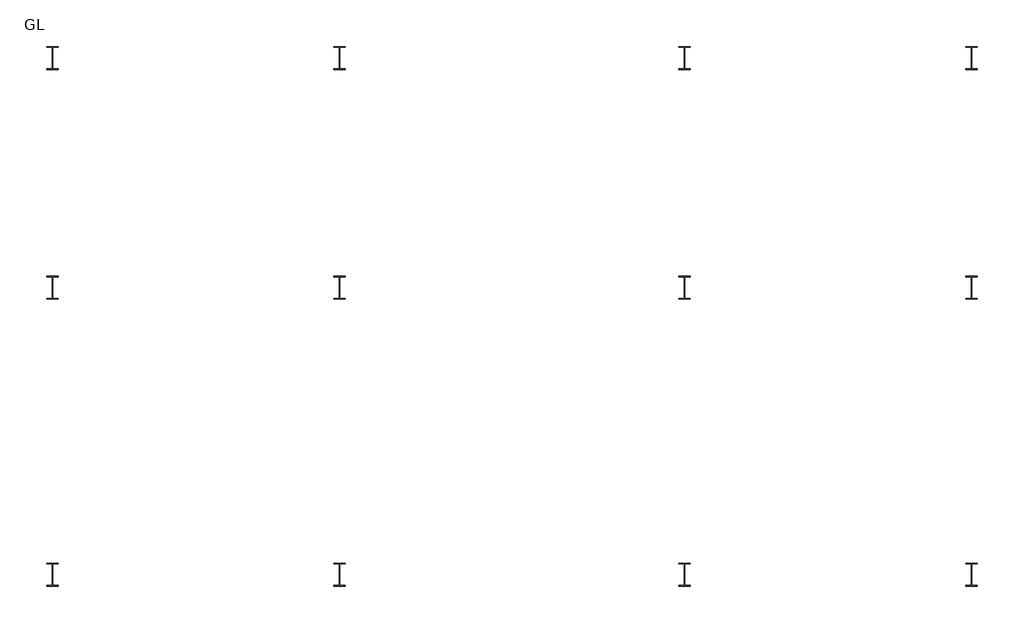
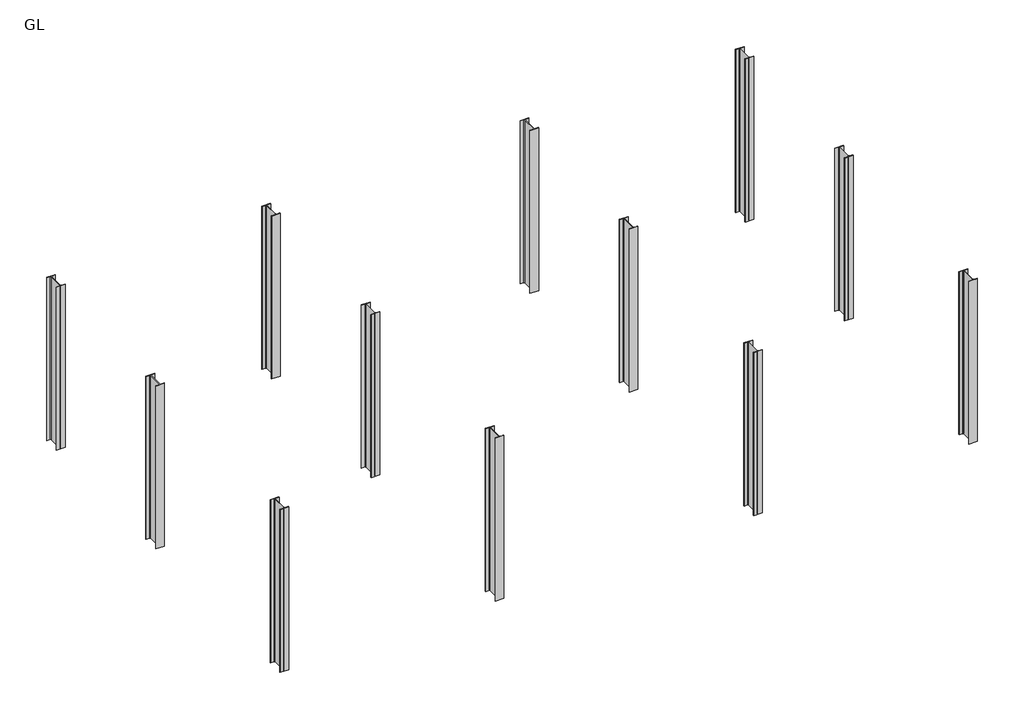
# One storey: 12 columns.
"""IFC4 building model written with IfcOpenShell, lengths in millimetres."""

from ifc_helpers import new_model, si_unit, point, frame_2d, origin, origin_with_axes, place, context, project, spatial, polyline, circle_curve, trimmed, segment, composite_curve, outline, extrude, element, save

model = new_model("IFC4")

# Units and contexts
model_context = context("Model", 3, world=origin())
ifc_project = project(units=[si_unit("LENGTHUNIT", "METRE", prefix="MILLI")], contexts=[model_context])

# Site, building, storey
site = spatial("IfcSite", under=ifc_project)
building = spatial("IfcBuilding", under=site)
storey = spatial("IfcBuildingStorey", under=building, Name="GL", Elevation=-0.0381366)

# Columns
placement = place(None, origin())
element("IfcColumn", 1, ObjectType="Steel Column_H_KSD3502 : H_SC_AR_S01_H-400x200x8x13", at=placement, inside=storey, context=model_context, shape_type="SweptSolid", body=[
    extrude(outline(composite_curve([segment(polyline([(100.0, 200.0), (100.0, 187.0), (20.0, 187.0)]), True, "CONTINUOUS"), segment(trimmed(circle_curve(frame_2d((20.0, 171.0)), 16.0), [point((20.0, 187.0))], [point((4.0, 171.0))], True, "CARTESIAN"), True, "CONTINUOUS"), segment(polyline([(4.0, 171.0), (4.0, -171.0)]), True, "CONTINUOUS"), segment(trimmed(circle_curve(frame_2d((20.0, -171.0)), 16.0), [point((4.0, -171.0))], [point((20.0, -187.0))], True, "CARTESIAN"), True, "CONTINUOUS"), segment(polyline([(20.0, -187.0), (100.0, -187.0), (100.0, -200.0), (-100.0, -200.0), (-100.0, -187.0), (-20.0, -187.0)]), True, "CONTINUOUS"), segment(trimmed(circle_curve(frame_2d((-20.0, -171.0)), 16.0), [point((-20.0, -187.0))], [point((-4.0, -171.0))], True, "CARTESIAN"), True, "CONTINUOUS"), segment(polyline([(-4.0, -171.0), (-4.0, 171.0)]), True, "CONTINUOUS"), segment(trimmed(circle_curve(frame_2d((-20.0, 171.0)), 16.0), [point((-4.0, 171.0))], [point((-20.0, 187.0))], True, "CARTESIAN"), True, "CONTINUOUS"), segment(polyline([(-20.0, 187.0), (-100.0, 187.0), (-100.0, 200.0), (100.0, 200.0)]), True, "CONTINUOUS")], self_intersect=False)), origin_with_axes(), (0.0, 0.0, 1.0), 4000.0),
])
element("IfcColumn", 2, ObjectType="Steel Column_H_KSD3502 : H_SC_AR_S01_H-400x200x8x13", at=placement, inside=storey, context=model_context, shape_type="SweptSolid", body=[
    extrude(outline(composite_curve([segment(polyline([(5100.0, 200.0), (5100.0, 187.0), (5020.0, 187.0)]), True, "CONTINUOUS"), segment(trimmed(circle_curve(frame_2d((5020.0, 171.0)), 16.0), [point((5020.0, 187.0))], [point((5004.0, 171.0))], True, "CARTESIAN"), True, "CONTINUOUS"), segment(polyline([(5004.0, 171.0), (5004.0, -171.0)]), True, "CONTINUOUS"), segment(trimmed(circle_curve(frame_2d((5020.0, -171.0)), 16.0), [point((5004.0, -171.0))], [point((5020.0, -187.0))], True, "CARTESIAN"), True, "CONTINUOUS"), segment(polyline([(5020.0, -187.0), (5100.0, -187.0), (5100.0, -200.0), (4900.0, -200.0), (4900.0, -187.0), (4980.0, -187.0)]), True, "CONTINUOUS"), segment(trimmed(circle_curve(frame_2d((4980.0, -171.0)), 16.0), [point((4980.0, -187.0))], [point((4996.0, -171.0))], True, "CARTESIAN"), True, "CONTINUOUS"), segment(polyline([(4996.0, -171.0), (4996.0, 171.0)]), True, "CONTINUOUS"), segment(trimmed(circle_curve(frame_2d((4980.0, 171.0)), 16.0), [point((4996.0, 171.0))], [point((4980.0, 187.0))], True, "CARTESIAN"), True, "CONTINUOUS"), segment(polyline([(4980.0, 187.0), (4900.0, 187.0), (4900.0, 200.0), (5100.0, 200.0)]), True, "CONTINUOUS")], self_intersect=False)), origin_with_axes(), (0.0, 0.0, 1.0), 4000.0),
])
element("IfcColumn", 3, ObjectType="Steel Column_H_KSD3502 : H_SC_AR_S01_H-400x200x8x13", at=placement, inside=storey, context=model_context, shape_type="SweptSolid", body=[
    extrude(outline(composite_curve([segment(polyline([(11100.0, 200.0), (11100.0, 187.0), (11020.0, 187.0)]), True, "CONTINUOUS"), segment(trimmed(circle_curve(frame_2d((11020.0, 171.0)), 16.0), [point((11020.0, 187.0))], [point((11004.0, 171.0))], True, "CARTESIAN"), True, "CONTINUOUS"), segment(polyline([(11004.0, 171.0), (11004.0, -171.0)]), True, "CONTINUOUS"), segment(trimmed(circle_curve(frame_2d((11020.0, -171.0)), 16.0), [point((11004.0, -171.0))], [point((11020.0, -187.0))], True, "CARTESIAN"), True, "CONTINUOUS"), segment(polyline([(11020.0, -187.0), (11100.0, -187.0), (11100.0, -200.0), (10900.0, -200.0), (10900.0, -187.0), (10980.0, -187.0)]), True, "CONTINUOUS"), segment(trimmed(circle_curve(frame_2d((10980.0, -171.0)), 16.0), [point((10980.0, -187.0))], [point((10996.0, -171.0))], True, "CARTESIAN"), True, "CONTINUOUS"), segment(polyline([(10996.0, -171.0), (10996.0, 171.0)]), True, "CONTINUOUS"), segment(trimmed(circle_curve(frame_2d((10980.0, 171.0)), 16.0), [point((10996.0, 171.0))], [point((10980.0, 187.0))], True, "CARTESIAN"), True, "CONTINUOUS"), segment(polyline([(10980.0, 187.0), (10900.0, 187.0), (10900.0, 200.0), (11100.0, 200.0)]), True, "CONTINUOUS")], self_intersect=False)), origin_with_axes(), (0.0, 0.0, 1.0), 4000.0),
])
element("IfcColumn", 4, ObjectType="Steel Column_H_KSD3502 : H_SC_AR_S01_H-400x200x8x13", at=placement, inside=storey, context=model_context, shape_type="SweptSolid", body=[
    extrude(outline(composite_curve([segment(polyline([(16100.0, 200.0), (16100.0, 187.0), (16020.0, 187.0)]), True, "CONTINUOUS"), segment(trimmed(circle_curve(frame_2d((16020.0, 171.0)), 16.0), [point((16020.0, 187.0))], [point((16004.0, 171.0))], True, "CARTESIAN"), True, "CONTINUOUS"), segment(polyline([(16004.0, 171.0), (16004.0, -171.0)]), True, "CONTINUOUS"), segment(trimmed(circle_curve(frame_2d((16020.0, -171.0)), 16.0), [point((16004.0, -171.0))], [point((16020.0, -187.0))], True, "CARTESIAN"), True, "CONTINUOUS"), segment(polyline([(16020.0, -187.0), (16100.0, -187.0), (16100.0, -200.0), (15900.0, -200.0), (15900.0, -187.0), (15980.0, -187.0)]), True, "CONTINUOUS"), segment(trimmed(circle_curve(frame_2d((15980.0, -171.0)), 16.0), [point((15980.0, -187.0))], [point((15996.0, -171.0))], True, "CARTESIAN"), True, "CONTINUOUS"), segment(polyline([(15996.0, -171.0), (15996.0, 171.0)]), True, "CONTINUOUS"), segment(trimmed(circle_curve(frame_2d((15980.0, 171.0)), 16.0), [point((15996.0, 171.0))], [point((15980.0, 187.0))], True, "CARTESIAN"), True, "CONTINUOUS"), segment(polyline([(15980.0, 187.0), (15900.0, 187.0), (15900.0, 200.0), (16100.0, 200.0)]), True, "CONTINUOUS")], self_intersect=False)), origin_with_axes(), (0.0, 0.0, 1.0), 4000.0),
])
element("IfcColumn", 5, ObjectType="Steel Column_H_KSD3502 : H_SC_AR_S01_H-400x200x8x13", at=placement, inside=storey, context=model_context, shape_type="SweptSolid", body=[
    extrude(outline(composite_curve([segment(polyline([(100.0, 5200.0), (100.0, 5187.0), (20.0, 5187.0)]), True, "CONTINUOUS"), segment(trimmed(circle_curve(frame_2d((20.0, 5171.0)), 16.0), [point((20.0, 5187.0))], [point((4.0, 5171.0))], True, "CARTESIAN"), True, "CONTINUOUS"), segment(polyline([(4.0, 5171.0), (4.0, 4829.0)]), True, "CONTINUOUS"), segment(trimmed(circle_curve(frame_2d((20.0, 4829.0)), 16.0), [point((4.0, 4829.0))], [point((20.0, 4813.0))], True, "CARTESIAN"), True, "CONTINUOUS"), segment(polyline([(20.0, 4813.0), (100.0, 4813.0), (100.0, 4800.0), (-100.0, 4800.0), (-100.0, 4813.0), (-20.0, 4813.0)]), True, "CONTINUOUS"), segment(trimmed(circle_curve(frame_2d((-20.0, 4829.0)), 16.0), [point((-20.0, 4813.0))], [point((-4.0, 4829.0))], True, "CARTESIAN"), True, "CONTINUOUS"), segment(polyline([(-4.0, 4829.0), (-4.0, 5171.0)]), True, "CONTINUOUS"), segment(trimmed(circle_curve(frame_2d((-20.0, 5171.0)), 16.0), [point((-4.0, 5171.0))], [point((-20.0, 5187.0))], True, "CARTESIAN"), True, "CONTINUOUS"), segment(polyline([(-20.0, 5187.0), (-100.0, 5187.0), (-100.0, 5200.0), (100.0, 5200.0)]), True, "CONTINUOUS")], self_intersect=False)), origin_with_axes(), (0.0, 0.0, 1.0), 4000.0),
])
element("IfcColumn", 6, ObjectType="Steel Column_H_KSD3502 : H_SC_AR_S01_H-400x200x8x13", at=placement, inside=storey, context=model_context, shape_type="SweptSolid", body=[
    extrude(outline(composite_curve([segment(polyline([(5100.0, 5200.0), (5100.0, 5187.0), (5020.0, 5187.0)]), True, "CONTINUOUS"), segment(trimmed(circle_curve(frame_2d((5020.0, 5171.0)), 16.0), [point((5020.0, 5187.0))], [point((5004.0, 5171.0))], True, "CARTESIAN"), True, "CONTINUOUS"), segment(polyline([(5004.0, 5171.0), (5004.0, 4829.0)]), True, "CONTINUOUS"), segment(trimmed(circle_curve(frame_2d((5020.0, 4829.0)), 16.0), [point((5004.0, 4829.0))], [point((5020.0, 4813.0))], True, "CARTESIAN"), True, "CONTINUOUS"), segment(polyline([(5020.0, 4813.0), (5100.0, 4813.0), (5100.0, 4800.0), (4900.0, 4800.0), (4900.0, 4813.0), (4980.0, 4813.0)]), True, "CONTINUOUS"), segment(trimmed(circle_curve(frame_2d((4980.0, 4829.0)), 16.0), [point((4980.0, 4813.0))], [point((4996.0, 4829.0))], True, "CARTESIAN"), True, "CONTINUOUS"), segment(polyline([(4996.0, 4829.0), (4996.0, 5171.0)]), True, "CONTINUOUS"), segment(trimmed(circle_curve(frame_2d((4980.0, 5171.0)), 16.0), [point((4996.0, 5171.0))], [point((4980.0, 5187.0))], True, "CARTESIAN"), True, "CONTINUOUS"), segment(polyline([(4980.0, 5187.0), (4900.0, 5187.0), (4900.0, 5200.0), (5100.0, 5200.0)]), True, "CONTINUOUS")], self_intersect=False)), origin_with_axes(), (0.0, 0.0, 1.0), 4000.0),
])
element("IfcColumn", 7, ObjectType="Steel Column_H_KSD3502 : H_SC_AR_S01_H-400x200x8x13", at=placement, inside=storey, context=model_context, shape_type="SweptSolid", body=[
    extrude(outline(composite_curve([segment(polyline([(11100.0, 5200.0), (11100.0, 5187.0), (11020.0, 5187.0)]), True, "CONTINUOUS"), segment(trimmed(circle_curve(frame_2d((11020.0, 5171.0)), 16.0), [point((11020.0, 5187.0))], [point((11004.0, 5171.0))], True, "CARTESIAN"), True, "CONTINUOUS"), segment(polyline([(11004.0, 5171.0), (11004.0, 4829.0)]), True, "CONTINUOUS"), segment(trimmed(circle_curve(frame_2d((11020.0, 4829.0)), 16.0), [point((11004.0, 4829.0))], [point((11020.0, 4813.0))], True, "CARTESIAN"), True, "CONTINUOUS"), segment(polyline([(11020.0, 4813.0), (11100.0, 4813.0), (11100.0, 4800.0), (10900.0, 4800.0), (10900.0, 4813.0), (10980.0, 4813.0)]), True, "CONTINUOUS"), segment(trimmed(circle_curve(frame_2d((10980.0, 4829.0)), 16.0), [point((10980.0, 4813.0))], [point((10996.0, 4829.0))], True, "CARTESIAN"), True, "CONTINUOUS"), segment(polyline([(10996.0, 4829.0), (10996.0, 5171.0)]), True, "CONTINUOUS"), segment(trimmed(circle_curve(frame_2d((10980.0, 5171.0)), 16.0), [point((10996.0, 5171.0))], [point((10980.0, 5187.0))], True, "CARTESIAN"), True, "CONTINUOUS"), segment(polyline([(10980.0, 5187.0), (10900.0, 5187.0), (10900.0, 5200.0), (11100.0, 5200.0)]), True, "CONTINUOUS")], self_intersect=False)), origin_with_axes(), (0.0, 0.0, 1.0), 4000.0),
])
element("IfcColumn", 8, ObjectType="Steel Column_H_KSD3502 : H_SC_AR_S01_H-400x200x8x13", at=placement, inside=storey, context=model_context, shape_type="SweptSolid", body=[
    extrude(outline(composite_curve([segment(polyline([(16100.0, 5200.0), (16100.0, 5187.0), (16020.0, 5187.0)]), True, "CONTINUOUS"), segment(trimmed(circle_curve(frame_2d((16020.0, 5171.0)), 16.0), [point((16020.0, 5187.0))], [point((16004.0, 5171.0))], True, "CARTESIAN"), True, "CONTINUOUS"), segment(polyline([(16004.0, 5171.0), (16004.0, 4829.0)]), True, "CONTINUOUS"), segment(trimmed(circle_curve(frame_2d((16020.0, 4829.0)), 16.0), [point((16004.0, 4829.0))], [point((16020.0, 4813.0))], True, "CARTESIAN"), True, "CONTINUOUS"), segment(polyline([(16020.0, 4813.0), (16100.0, 4813.0), (16100.0, 4800.0), (15900.0, 4800.0), (15900.0, 4813.0), (15980.0, 4813.0)]), True, "CONTINUOUS"), segment(trimmed(circle_curve(frame_2d((15980.0, 4829.0)), 16.0), [point((15980.0, 4813.0))], [point((15996.0, 4829.0))], True, "CARTESIAN"), True, "CONTINUOUS"), segment(polyline([(15996.0, 4829.0), (15996.0, 5171.0)]), True, "CONTINUOUS"), segment(trimmed(circle_curve(frame_2d((15980.0, 5171.0)), 16.0), [point((15996.0, 5171.0))], [point((15980.0, 5187.0))], True, "CARTESIAN"), True, "CONTINUOUS"), segment(polyline([(15980.0, 5187.0), (15900.0, 5187.0), (15900.0, 5200.0), (16100.0, 5200.0)]), True, "CONTINUOUS")], self_intersect=False)), origin_with_axes(), (0.0, 0.0, 1.0), 4000.0),
])
element("IfcColumn", 9, ObjectType="Steel Column_H_KSD3502 : H_SC_AR_S01_H-400x200x8x13", at=placement, inside=storey, context=model_context, shape_type="SweptSolid", body=[
    extrude(outline(composite_curve([segment(polyline([(100.0, 9200.0), (100.0, 9187.0), (20.0, 9187.0)]), True, "CONTINUOUS"), segment(trimmed(circle_curve(frame_2d((20.0, 9171.0)), 16.0), [point((20.0, 9187.0))], [point((4.0, 9171.0))], True, "CARTESIAN"), True, "CONTINUOUS"), segment(polyline([(4.0, 9171.0), (4.0, 8829.0)]), True, "CONTINUOUS"), segment(trimmed(circle_curve(frame_2d((20.0, 8829.0)), 16.0), [point((4.0, 8829.0))], [point((20.0, 8813.0))], True, "CARTESIAN"), True, "CONTINUOUS"), segment(polyline([(20.0, 8813.0), (100.0, 8813.0), (100.0, 8800.0), (-100.0, 8800.0), (-100.0, 8813.0), (-20.0, 8813.0)]), True, "CONTINUOUS"), segment(trimmed(circle_curve(frame_2d((-20.0, 8829.0)), 16.0), [point((-20.0, 8813.0))], [point((-4.0, 8829.0))], True, "CARTESIAN"), True, "CONTINUOUS"), segment(polyline([(-4.0, 8829.0), (-4.0, 9171.0)]), True, "CONTINUOUS"), segment(trimmed(circle_curve(frame_2d((-20.0, 9171.0)), 16.0), [point((-4.0, 9171.0))], [point((-20.0, 9187.0))], True, "CARTESIAN"), True, "CONTINUOUS"), segment(polyline([(-20.0, 9187.0), (-100.0, 9187.0), (-100.0, 9200.0), (100.0, 9200.0)]), True, "CONTINUOUS")], self_intersect=False)), origin_with_axes(), (0.0, 0.0, 1.0), 4000.0),
])
element("IfcColumn", 10, ObjectType="Steel Column_H_KSD3502 : H_SC_AR_S01_H-400x200x8x13", at=placement, inside=storey, context=model_context, shape_type="SweptSolid", body=[
    extrude(outline(composite_curve([segment(polyline([(5100.0, 9200.0), (5100.0, 9187.0), (5020.0, 9187.0)]), True, "CONTINUOUS"), segment(trimmed(circle_curve(frame_2d((5020.0, 9171.0)), 16.0), [point((5020.0, 9187.0))], [point((5004.0, 9171.0))], True, "CARTESIAN"), True, "CONTINUOUS"), segment(polyline([(5004.0, 9171.0), (5004.0, 8829.0)]), True, "CONTINUOUS"), segment(trimmed(circle_curve(frame_2d((5020.0, 8829.0)), 16.0), [point((5004.0, 8829.0))], [point((5020.0, 8813.0))], True, "CARTESIAN"), True, "CONTINUOUS"), segment(polyline([(5020.0, 8813.0), (5100.0, 8813.0), (5100.0, 8800.0), (4900.0, 8800.0), (4900.0, 8813.0), (4980.0, 8813.0)]), True, "CONTINUOUS"), segment(trimmed(circle_curve(frame_2d((4980.0, 8829.0)), 16.0), [point((4980.0, 8813.0))], [point((4996.0, 8829.0))], True, "CARTESIAN"), True, "CONTINUOUS"), segment(polyline([(4996.0, 8829.0), (4996.0, 9171.0)]), True, "CONTINUOUS"), segment(trimmed(circle_curve(frame_2d((4980.0, 9171.0)), 16.0), [point((4996.0, 9171.0))], [point((4980.0, 9187.0))], True, "CARTESIAN"), True, "CONTINUOUS"), segment(polyline([(4980.0, 9187.0), (4900.0, 9187.0), (4900.0, 9200.0), (5100.0, 9200.0)]), True, "CONTINUOUS")], self_intersect=False)), origin_with_axes(), (0.0, 0.0, 1.0), 4000.0),
])
element("IfcColumn", 11, ObjectType="Steel Column_H_KSD3502 : H_SC_AR_S01_H-400x200x8x13", at=placement, inside=storey, context=model_context, shape_type="SweptSolid", body=[
    extrude(outline(composite_curve([segment(polyline([(11100.0, 9200.0), (11100.0, 9187.0), (11020.0, 9187.0)]), True, "CONTINUOUS"), segment(trimmed(circle_curve(frame_2d((11020.0, 9171.0)), 16.0), [point((11020.0, 9187.0))], [point((11004.0, 9171.0))], True, "CARTESIAN"), True, "CONTINUOUS"), segment(polyline([(11004.0, 9171.0), (11004.0, 8829.0)]), True, "CONTINUOUS"), segment(trimmed(circle_curve(frame_2d((11020.0, 8829.0)), 16.0), [point((11004.0, 8829.0))], [point((11020.0, 8813.0))], True, "CARTESIAN"), True, "CONTINUOUS"), segment(polyline([(11020.0, 8813.0), (11100.0, 8813.0), (11100.0, 8800.0), (10900.0, 8800.0), (10900.0, 8813.0), (10980.0, 8813.0)]), True, "CONTINUOUS"), segment(trimmed(circle_curve(frame_2d((10980.0, 8829.0)), 16.0), [point((10980.0, 8813.0))], [point((10996.0, 8829.0))], True, "CARTESIAN"), True, "CONTINUOUS"), segment(polyline([(10996.0, 8829.0), (10996.0, 9171.0)]), True, "CONTINUOUS"), segment(trimmed(circle_curve(frame_2d((10980.0, 9171.0)), 16.0), [point((10996.0, 9171.0))], [point((10980.0, 9187.0))], True, "CARTESIAN"), True, "CONTINUOUS"), segment(polyline([(10980.0, 9187.0), (10900.0, 9187.0), (10900.0, 9200.0), (11100.0, 9200.0)]), True, "CONTINUOUS")], self_intersect=False)), origin_with_axes(), (0.0, 0.0, 1.0), 4000.0),
])
element("IfcColumn", 12, ObjectType="Steel Column_H_KSD3502 : H_SC_AR_S01_H-400x200x8x13", at=placement, inside=storey, context=model_context, shape_type="SweptSolid", body=[
    extrude(outline(composite_curve([segment(polyline([(16100.0, 9200.0), (16100.0, 9187.0), (16020.0, 9187.0)]), True, "CONTINUOUS"), segment(trimmed(circle_curve(frame_2d((16020.0, 9171.0)), 16.0), [point((16020.0, 9187.0))], [point((16004.0, 9171.0))], True, "CARTESIAN"), True, "CONTINUOUS"), segment(polyline([(16004.0, 9171.0), (16004.0, 8829.0)]), True, "CONTINUOUS"), segment(trimmed(circle_curve(frame_2d((16020.0, 8829.0)), 16.0), [point((16004.0, 8829.0))], [point((16020.0, 8813.0))], True, "CARTESIAN"), True, "CONTINUOUS"), segment(polyline([(16020.0, 8813.0), (16100.0, 8813.0), (16100.0, 8800.0), (15900.0, 8800.0), (15900.0, 8813.0), (15980.0, 8813.0)]), True, "CONTINUOUS"), segment(trimmed(circle_curve(frame_2d((15980.0, 8829.0)), 16.0), [point((15980.0, 8813.0))], [point((15996.0, 8829.0))], True, "CARTESIAN"), True, "CONTINUOUS"), segment(polyline([(15996.0, 8829.0), (15996.0, 9171.0)]), True, "CONTINUOUS"), segment(trimmed(circle_curve(frame_2d((15980.0, 9171.0)), 16.0), [point((15996.0, 9171.0))], [point((15980.0, 9187.0))], True, "CARTESIAN"), True, "CONTINUOUS"), segment(polyline([(15980.0, 9187.0), (15900.0, 9187.0), (15900.0, 9200.0), (16100.0, 9200.0)]), True, "CONTINUOUS")], self_intersect=False)), origin_with_axes(), (0.0, 0.0, 1.0), 4000.0),
])

save(model, "model.ifc")

# Revit data of these elements
# Project information
#   H_Seismic Condition = "A as per ASCE 7-10"
#   H_Soil Condition = "C as per ASCE 7-10"
#   H_Basic Wind Speed = "58.3m/s ASCE7-10"
#   H_DS Project Code = "FAASA2302"
#   H_Project Abbreviation = "SACE2"
#   H_Project Division = "화공"
#   H_Project Finish = "2027-03-05"
#   H_Project Location = "Jafurah, Saudi Arabia"
#   H_Project Start = "2024-01-03"
#   H_Project Type = "EPC"
#   H_Smart Code = "FAASA2302"
#   Project Issue Date = "Issue Date"
#   Project Status = "Project Status"
#   Client Name = "Owner"
#   Project Address = "Enter address here"
#   Project Name = "Project Name"
#   Project Number = "0001"
# Grids (mm)
#   "A": line (-3000, 0) -> (19000, 0)
#   "B": line (-3000, 5000) -> (19000, 5000)
#   "C": line (-3000, 9000) -> (19000, 9000)
#   "1": line (0, -3000) -> (0, 12000)
#   "2": line (5000, -3000) -> (5000, 12000)
#   "3": line (11000, -3000) -> (11000, 12000)
#   "4": line (16000, -3000) -> (16000, 12000)
# Type "Steel Column_H_KSD3502 : H_SC_AR_S01_H-400x200x8x13"
#   Width = 20.0 cm
#   Web Thickness = 0.8 cm
#   Web Fillet = 1.6 cm
#   Warping Constant = 648999.0 cm⁶
#   Torsional Moment of Inertia = 35.8981 cm⁴
#   Section Area = 84.12 cm²
#   Plastic Modulus weak axis = 268.0 cm³
#   Plastic Modulus strong axis = 1330.0 cm³
#   Perimeter = 1.56 m²/m
#   Nominal Weight = 66.00 kgf/m
#   Moment of Inertia weak axis = 1740.00 cm⁴
#   Moment of Inertia strong axis = 23700.00 cm⁴
#   Height = 40.0 cm
#   Flange Thickness = 1.3 cm
#   Elastic Modulus weak axis = 174.0 cm³
#   Elastic Modulus strong axis = 1190.0 cm³
#   Centroid Vertical = 20.0 cm
#   Centroid Horizontal = 10.0 cm
#   Structural Material [instance default] = Steel, 45-345
#   Section Name Key = ""
#   Bolt Spacing = 0
#   Assembly Code = ""
# Elements 1, 2, 3, 4, 5, 6, 7, 8, 9, 10, 11, 12 (IfcColumn, "Steel Column_H_KSD3502 : H_SC_AR_S01_H-400x200x8x13")
#   Comments = ""
#   HSD_member_analysis = ""
#   Structural Material = none
#   Phase Created = New Construction
# Materials
#   "Steel, 45-345": class "Metal", colour RGB 189 187 185, transparency 0, Description = "Steel 345 MPa", Cost = 0
